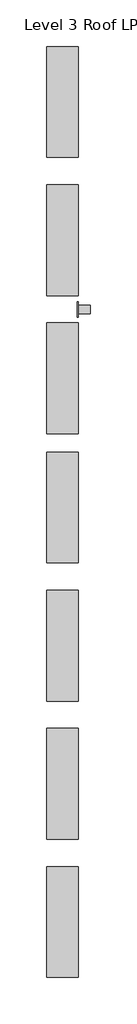
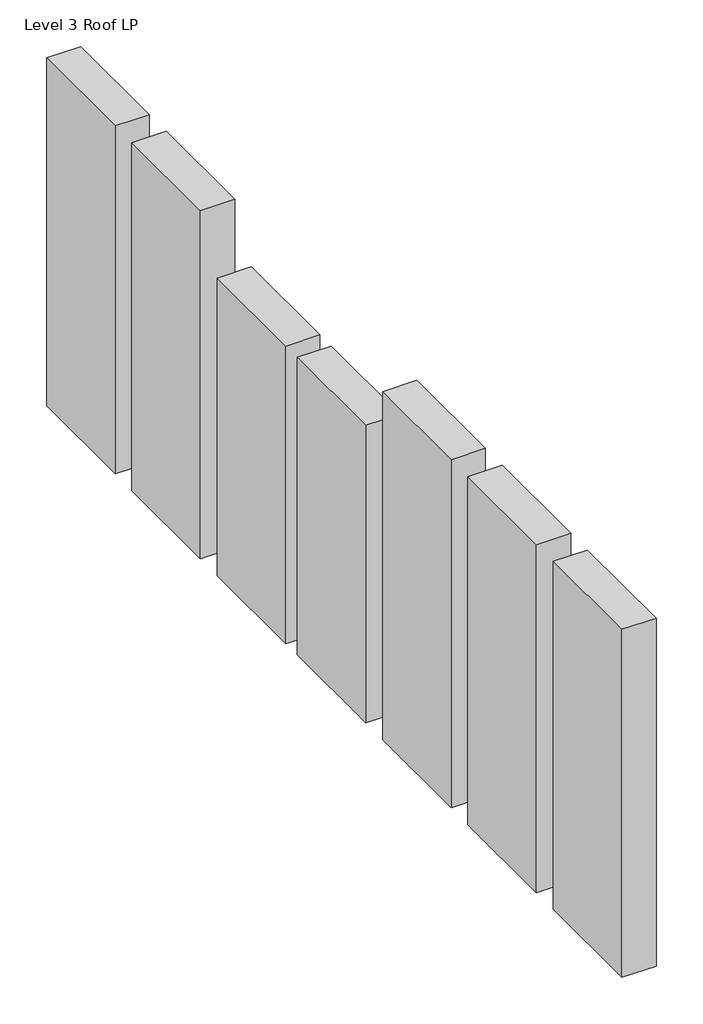
# One storey: 8 proxies.
"""IFC4 building model written with IfcOpenShell, lengths in millimetres."""

import ifcopenshell
import ifcopenshell.guid

model = None  # the IFC model being written
_history = None  # IfcOwnerHistory: only IFC2X3 demands one
_inside = {}  # id of a spatial element -> (the spatial element, [elements in it])
_under = {}  # id of a project, library or spatial element -> (it, [spatial elements below it])
_declared = {}  # id of a project -> (the project, [libraries it declares])
_typed = {}  # id of a type object -> (the type object, [elements of that type])
_made_of = {}  # id of a material, layer set ... -> (it, [elements and type objects made of it])


def new_model(schema):
    """Start an empty IFC model of exactly this schema.

    Asked for "IFC4X3", IfcOpenShell would pick the latest addendum, in which some entities
    have other attributes; the version numbers below select the first issue.
    IFC2X3 requires an IfcOwnerHistory on every rooted entity: one is made here for all.
    """
    global model, _history
    if schema == "IFC4X3":
        model = ifcopenshell.file(schema_version=(4, 3, 0, 0))
    else:
        model = ifcopenshell.file(schema=schema)
    _inside.clear()
    _under.clear()
    _declared.clear()
    _typed.clear()
    _made_of.clear()
    _history = None
    if model.schema == "IFC2X3":
        org = make("IfcOrganization", Name="unknown")
        user = make(
            "IfcPersonAndOrganization",
            ThePerson=make("IfcPerson", FamilyName="unknown"),
            TheOrganization=org,
        )
        app = make(
            "IfcApplication",
            ApplicationDeveloper=org,
            Version="unknown",
            ApplicationFullName="unknown",
            ApplicationIdentifier="unknown",
        )
        _history = make(
            "IfcOwnerHistory",
            OwningUser=user,
            OwningApplication=app,
            ChangeAction="ADDED",
            CreationDate=0,
        )
    return model


def make(cls, **values):
    """One entity of the class cls with the attributes given. An attribute that is None is left unset."""
    return model.create_entity(
        cls, **{name: value for name, value in values.items() if value is not None}
    )


def rooted(cls, **values):
    """An entity with a GlobalId (a new one), such as an element, a storey or a relation."""
    return make(cls, GlobalId=ifcopenshell.guid.new(), OwnerHistory=_history, **values)


def si_unit(unit_type, name, prefix=None):
    """IfcSIUnit, for example si_unit("LENGTHUNIT", "METRE", prefix="MILLI")."""
    return make("IfcSIUnit", UnitType=unit_type, Prefix=prefix, Name=name)


def assignment(units):
    """IfcUnitAssignment: the units of a project."""
    return None if units is None else make("IfcUnitAssignment", Units=units)


def point(xyz):
    """IfcCartesianPoint."""
    return None if xyz is None else make("IfcCartesianPoint", Coordinates=xyz)


def direction(xyz):
    """IfcDirection."""
    return None if xyz is None else make("IfcDirection", DirectionRatios=xyz)


def frame(location, z_axis=None, x_axis=None):
    """IfcAxis2Placement3D, a coordinate frame: its origin and axes. An axis left out is left unset."""
    return make(
        "IfcAxis2Placement3D",
        Location=point(location),
        Axis=direction(z_axis),
        RefDirection=direction(x_axis),
    )


def origin():
    """The frame at (0, 0, 0) with its axes left unset."""
    return frame((0.0, 0.0, 0.0))


def origin_with_axes():
    """The frame at (0, 0, 0) with the z axis (0, 0, 1) and the x axis (1, 0, 0) written out."""
    return frame((0.0, 0.0, 0.0), z_axis=(0.0, 0.0, 1.0), x_axis=(1.0, 0.0, 0.0))


def place(relative_to, where):
    """IfcLocalPlacement: puts the frame where relative to a parent placement (None: the world)."""
    return make(
        "IfcLocalPlacement", PlacementRelTo=relative_to, RelativePlacement=where
    )


def context(
    kind, dimensions, precision=None, world=None, true_north=None, identifier=None
):
    """IfcGeometricRepresentationContext, for example the 3D "Model" context."""
    return make(
        "IfcGeometricRepresentationContext",
        ContextIdentifier=identifier,
        ContextType=kind,
        CoordinateSpaceDimension=dimensions,
        Precision=precision,
        WorldCoordinateSystem=world,
        TrueNorth=true_north,
    )


def project(units=None, contexts=None):
    """IfcProject with its units and contexts."""
    return rooted(
        "IfcProject",
        Name="project",
        RepresentationContexts=contexts,
        UnitsInContext=assignment(units),
    )


def spatial(cls, under=None, at=None, **own):
    """A site, building, storey or space (cls), placed at a placement, below another one or the project."""
    s = rooted(cls, ObjectPlacement=at, **own)
    if under is not None:
        _under.setdefault(under.id(), (under, []))[1].append(s)
    return s


def polyline(points):
    """IfcPolyline through the points."""
    return make("IfcPolyline", Points=[point(p) for p in points])


def outline(outer, holes=None, kind="AREA"):
    """IfcArbitraryClosedProfileDef: a profile drawn as a closed curve; with holes, ...WithVoids."""
    if holes is None:
        return make("IfcArbitraryClosedProfileDef", ProfileType=kind, OuterCurve=outer)
    return make(
        "IfcArbitraryProfileDefWithVoids",
        ProfileType=kind,
        OuterCurve=outer,
        InnerCurves=holes,
    )


def extrude(swept, where, along, depth):
    """IfcExtrudedAreaSolid: the profile swept, set in the frame where, extruded along a direction by depth."""
    return make(
        "IfcExtrudedAreaSolid",
        SweptArea=swept,
        Position=where,
        ExtrudedDirection=direction(along),
        Depth=depth,
    )


def shape(context_of_items, identifier, shape_type, items):
    """IfcShapeRepresentation: the items that make up one representation, for example the "Body"."""
    return make(
        "IfcShapeRepresentation",
        ContextOfItems=context_of_items,
        RepresentationIdentifier=identifier,
        RepresentationType=shape_type,
        Items=items,
    )


def source(mapping_origin, context_of_items, identifier, shape_type, items):
    """IfcRepresentationMap: a shape defined once, which mapped items show again and again."""
    return make(
        "IfcRepresentationMap",
        MappingOrigin=mapping_origin,
        MappedRepresentation=shape(context_of_items, identifier, shape_type, items),
    )


def transform(
    local_origin,
    x_axis=None,
    y_axis=None,
    z_axis=None,
    scale=None,
    scale2=None,
    scale3=None,
    uniform=True,
):
    """IfcCartesianTransformationOperator3D, or its non-uniform kind. x_axis, y_axis, z_axis: its Axis1, 2, 3."""
    if uniform:
        return make(
            "IfcCartesianTransformationOperator3D",
            Axis1=direction(x_axis),
            Axis2=direction(y_axis),
            LocalOrigin=point(local_origin),
            Scale=scale,
            Axis3=direction(z_axis),
        )
    return make(
        "IfcCartesianTransformationOperator3DnonUniform",
        Axis1=direction(x_axis),
        Axis2=direction(y_axis),
        LocalOrigin=point(local_origin),
        Scale=scale,
        Axis3=direction(z_axis),
        Scale2=scale2,
        Scale3=scale3,
    )


def mapped(mapping_source, mapping_target):
    """IfcMappedItem: shows the shape of a source again, moved by a transform."""
    return make(
        "IfcMappedItem", MappingSource=mapping_source, MappingTarget=mapping_target
    )


def made_of(thing, what):
    """Note that an element or type object is made of a material, layer set ...; save() writes the relation."""
    if what is not None:
        _made_of.setdefault(what.id(), (what, []))[1].append(thing)
    return thing


def element(
    cls,
    number,
    at=None,
    inside=None,
    cuts=None,
    type_object=None,
    material=None,
    context=None,
    identifier="Body",
    shape_type=None,
    held_by="IfcProductDefinitionShape",
    body=None,
    shapes=None,
    **own,
):
    """One element of the class cls, such as IfcWall. Its Tag is "e" and its number.

    at: its placement. inside: the storey or other place that contains it. cuts: it is an
    opening in that element (IfcRelVoidsElement). A single representation is given by context,
    identifier, shape_type and body (its items); several are given by shapes. held_by: the class
    of the entity that holds the representations. save() writes the other relations.
    """
    e = rooted(cls, Tag="e%d" % number, ObjectPlacement=at, **own)
    if body is not None:
        shapes = [shape(context, identifier, shape_type, body)]
    if shapes is not None:
        e.Representation = make(held_by, Representations=shapes)
    if inside is not None:
        _inside.setdefault(inside.id(), (inside, []))[1].append(e)
    if cuts is not None:
        rooted(
            "IfcRelVoidsElement", RelatingBuildingElement=cuts, RelatedOpeningElement=e
        )
    if type_object is not None:
        _typed.setdefault(type_object.id(), (type_object, []))[1].append(e)
    return made_of(e, material)


def aggregate(whole, parts):
    """IfcRelAggregates: a whole, such as a stair, and the parts it consists of."""
    return rooted("IfcRelAggregates", RelatingObject=whole, RelatedObjects=parts)


def save(model, path):
    """Write the relations noted so far, then the file.

    IfcRelAggregates (storeys below a building ...), IfcRelContainedInSpatialStructure (elements
    in a storey), IfcRelDefinesByType, IfcRelAssociatesMaterial and IfcRelDeclares: one each for
    every whole, place, type object, material and project.
    """
    for whole, parts in _under.values():
        aggregate(whole, parts)
    for where, things in _inside.values():
        rooted(
            "IfcRelContainedInSpatialStructure",
            RelatedElements=things,
            RelatingStructure=where,
        )
    for kind, things in _typed.values():
        rooted("IfcRelDefinesByType", RelatedObjects=things, RelatingType=kind)
    for what, things in _made_of.values():
        rooted("IfcRelAssociatesMaterial", RelatedObjects=things, RelatingMaterial=what)
    for by, libraries in _declared.values():
        rooted("IfcRelDeclares", RelatingContext=by, RelatedDefinitions=libraries)
    model.write(path)


def emergency_lighting_distribution_board_600_a_cf68ca70(model_context):
    return source(origin(), model_context, "Body", "SweptSolid", [
        extrude(outline(polyline([(254.0, -1346.2), (-254.0, -1346.2), (-254.0, 0.0), (254.0, 0.0), (254.0, -1346.2)])), origin_with_axes(), (0.0, 0.0, 1.0), 146.1),
    ])


def lighting_and_appliance_panelboard_400v_mcb_surface_400_a_826206d9(model_context):
    return source(origin(), model_context, "Body", "SweptSolid", [
        extrude(outline(polyline([(254.0, -1574.8), (-254.0, -1574.8), (-254.0, 0.0), (254.0, 0.0), (254.0, -1574.8)])), origin_with_axes(), (0.0, 0.0, 1.0), 146.1),
    ])


def m_duplex_receptacle_top_switched_standard_10251bba(model_context):
    return source(origin(), model_context, "Body", "SweptSolid", [
        extrude(outline(polyline([(19.05, 38.1), (19.05, -38.1), (-19.05, -38.1), (-19.05, 38.1), (19.05, 38.1)])), frame((0.0, 0.0, -53.975), z_axis=(0.0, 0.0, 1.0), x_axis=(1.0, 0.0, 0.0)), (0.0, 0.0, 1.0), 53.975),
        extrude(outline(polyline([(34.925, 57.15), (34.925, -57.15), (-34.925, -57.15), (-34.925, 57.15), (34.925, 57.15)])), origin_with_axes(), (0.0, 0.0, 1.0), 4.7625),
    ])


model = new_model("IFC4")

# Units and contexts
model_context = context("Model", 3, world=origin())
ifc_project = project(units=[si_unit("LENGTHUNIT", "METRE", prefix="MILLI")], contexts=[model_context])

# Site, building, storey
site = spatial("IfcSite", under=ifc_project)
building = spatial("IfcBuilding", under=site)
storey = spatial("IfcBuildingStorey", under=building, Name="Level 3 Roof LP", Elevation=107300.0)

# Proxies
placement = place(None, origin())
emergency_lighting_distribution_board_600_a_shape = emergency_lighting_distribution_board_600_a_cf68ca70(model_context)
element("IfcBuildingElementProxy", 1, Name="Emergency Lighting Distribution Board : 600 A", ObjectType="Emergency Lighting Distribution Board : 600 A", at=placement, inside=storey, context=model_context, shape_type="MappedRepresentation", body=[
    mapped(emergency_lighting_distribution_board_600_a_shape, transform((15990.005, 12707.4241924, 101351.4), x_axis=(0.0, -1.0, 0.0), y_axis=(0.0, 0.0, 1.0), z_axis=(-1.0, 0.0, 0.0))),
])
element("IfcBuildingElementProxy", 2, Name="Emergency Lighting Distribution Board : 600 A", ObjectType="Emergency Lighting Distribution Board : 600 A", at=placement, inside=storey, context=model_context, shape_type="MappedRepresentation", body=[
    mapped(emergency_lighting_distribution_board_600_a_shape, transform((15990.005, 13299.4241924, 101351.4), x_axis=(0.0, -1.0, 0.0), y_axis=(0.0, 0.0, 1.0), z_axis=(-1.0, 0.0, 0.0))),
])
lighting_and_appliance_panelboard_400v_mcb_surface_400_a_shape = lighting_and_appliance_panelboard_400v_mcb_surface_400_a_826206d9(model_context)
element("IfcBuildingElementProxy", 3, Name="Lighting and Appliance Panelboard - 400V MCB - Surface : 400 A", ObjectType="Lighting and Appliance Panelboard - 400V MCB - Surface : 400 A", at=placement, inside=storey, context=model_context, shape_type="MappedRepresentation", body=[
    mapped(lighting_and_appliance_panelboard_400v_mcb_surface_400_a_shape, transform((15990.005, 10808.4241924, 101580.0), x_axis=(0.0, -1.0, 0.0), y_axis=(0.0, 0.0, 1.0), z_axis=(-1.0, 0.0, 0.0))),
])
element("IfcBuildingElementProxy", 4, Name="Lighting and Appliance Panelboard - 400V MCB - Surface : 400 A", ObjectType="Lighting and Appliance Panelboard - 400V MCB - Surface : 400 A", at=placement, inside=storey, context=model_context, shape_type="MappedRepresentation", body=[
    mapped(lighting_and_appliance_panelboard_400v_mcb_surface_400_a_shape, transform((15990.005, 11441.4241924, 101580.0), x_axis=(0.0, -1.0, 0.0), y_axis=(0.0, 0.0, 1.0), z_axis=(-1.0, 0.0, 0.0))),
])
element("IfcBuildingElementProxy", 5, Name="Lighting and Appliance Panelboard - 400V MCB - Surface : 400 A", ObjectType="Lighting and Appliance Panelboard - 400V MCB - Surface : 400 A", at=placement, inside=storey, context=model_context, shape_type="MappedRepresentation", body=[
    mapped(lighting_and_appliance_panelboard_400v_mcb_surface_400_a_shape, transform((15990.005, 12074.4241924, 101580.0), x_axis=(0.0, -1.0, 0.0), y_axis=(0.0, 0.0, 1.0), z_axis=(-1.0, 0.0, 0.0))),
])
element("IfcBuildingElementProxy", 6, Name="Lighting and Appliance Panelboard - 400V MCB - Surface : 400 A", ObjectType="Lighting and Appliance Panelboard - 400V MCB - Surface : 400 A", at=placement, inside=storey, context=model_context, shape_type="MappedRepresentation", body=[
    mapped(lighting_and_appliance_panelboard_400v_mcb_surface_400_a_shape, transform((15990.005, 13932.4241924, 101580.0), x_axis=(0.0, -1.0, 0.0), y_axis=(0.0, 0.0, 1.0), z_axis=(-1.0, 0.0, 0.0))),
])
element("IfcBuildingElementProxy", 7, Name="Lighting and Appliance Panelboard - 400V MCB - Surface : 400 A", ObjectType="Lighting and Appliance Panelboard - 400V MCB - Surface : 400 A", at=placement, inside=storey, context=model_context, shape_type="MappedRepresentation", body=[
    mapped(lighting_and_appliance_panelboard_400v_mcb_surface_400_a_shape, transform((15990.005, 14565.4241924, 101580.0), x_axis=(0.0, -1.0, 0.0), y_axis=(0.0, 0.0, 1.0), z_axis=(-1.0, 0.0, 0.0))),
])
m_duplex_receptacle_top_switched_standard_shape = m_duplex_receptacle_top_switched_standard_10251bba(model_context)
element("IfcBuildingElementProxy", 8, Name="M_Receptacle - 220V : Standard", ObjectType="M_Receptacle - 220V : Standard", at=placement, inside=storey, context=model_context, shape_type="MappedRepresentation", body=[
    mapped(m_duplex_receptacle_top_switched_standard_shape, transform((15990.005, 13614.2932067, 100325.120044), x_axis=(0.0, -1.0, 0.0), y_axis=(0.0, 0.0, 1.0), z_axis=(-1.0, 0.0, 0.0))),
])

save(model, "model.ifc")

# Revit data of these elements
# Type "Emergency Lighting Distribution Board : 600 A"
#   Type Mark = "Emergency Lighting Distribution Board"
#   Classification.OmniClass.21.Number = "21-04 50 40 50"
#   Classification.OmniClass.21.Description = "Lighting Fixtures"
#   Classification.UniFormat.II.Description = "Lighting Fixtures"
#   Classification.OmniClass.23.Number = "23-35 31 13"
#   Classification.OmniClass.23.Description = "Distribution Panel Boards"
#   Classification.UniFormat.II.Number = "D5040.50"
#   COBie.Type.CreatedBy = "info@mma.ie"
#   COBie.Type.CreatedOn = "2017-07-25T10:15:16"
#   COBie.Type.Name = "Emergency Lighting Distribution Board"
#   COBie.Type.Category = "23-35 31 13 : Distribution Panel Boards"
#   COBie.Type.Description = "Emergency Lighting Distribution Board_600 A"
#   COBie.Type.AssetType = "Fixed"
#   COBie.Type.Manufacturer = ""
#   COBie.Type.ModelNumber = ""
#   Wattage = "400"
#   Voltage = "600"
#   built-in parameter 1140081 [instance default] = "Recessed"
#   Keynote = "26 26 00.A"
#   built-in parameter 1140083 [instance default] = "Type 1"
#   COBie.Type.ReplacementCost = 0
#   Width = 508 mm
#   built-in parameter 1140082 [instance default] = 100 (stored number, unit not read)
#   built-in parameter 1140140 [instance default] = 600 (stored number, unit not read)
#   Height [instance default] = 1346.2 mm
#   ELDB Width = 508 mm
#   ELDB Height = 1346.2 mm
#   ELDB Depth = 146.1 mm
#   Depth = 146.1 mm
#   Default Elevation = 1200 mm
#   Ballast Wattage = 400 W
#   Ballast Voltage = 600 V
#   42 Circuit Height = 1879.6 mm
#   30 Circuit Height = 1651 mm
#   24 Circuit Height = 1346.2 mm
#   12 Circuit Height = 1346.2 mm
#   COBie.Type = yes
#   built-in parameter 1140142 [instance default] = -1
#   built-in parameter 1140079 [instance default] = 12
#   built-in parameter 1155100 [instance default] = -1
#   Load Classification = Other
# Type "Lighting and Appliance Panelboard - 400V MCB - Surface : 400 A"
#   Type Mark = "Lighting and Appliance Panelboard - 400V MCB - Surface"
#   Classification.OmniClass.21.Number = "21-04 50 30 50"
#   Classification.MasterFormat.Description = "Wiring Devices"
#   Classification.OmniClass.22.Number = "22-26 27 26"
#   Classification.OmniClass.21.Description = "Wiring Devices"
#   Classification.UniFormat.II.Description = "Wiring Devices"
#   Classification.MasterFormat.Number = "26 27 26"
#   Classification.OmniClass.23.Number = "23-35 31 29"
#   Classification.OmniClass.22.Description = "Wiring Devices"
#   Classification.OmniClass.23.Description = "Switchboards"
#   Classification.UniFormat.II.Number = "D5030.50"
#   COBie.Type.CreatedBy = "info@mma.ie"
#   COBie.Type.CreatedOn = "2017-07-25T10:15:16"
#   COBie.Type.Name = "Lighting and Appliance Panelboard - 400V MCB - Surface"
#   COBie.Type.Category = "23-35 31 29 : Switchboards"
#   COBie.Type.Description = "Lighting and Appliance Panelboard - 400V MCB - Surface_400 A"
#   COBie.Type.AssetType = "Fixed"
#   COBie.Type.Manufacturer = ""
#   COBie.Type.ModelNumber = ""
#   Wattage = "400"
#   Voltage = "600"
#   built-in parameter 1140081 [instance default] = "Surface"
#   Keynote = "26 24 16.A"
#   built-in parameter 1140083 [instance default] = "Type 1"
#   COBie.Type.ReplacementCost = 0
#   Width = 508 mm
#   built-in parameter 1140082 [instance default] = 100 (stored number, unit not read)
#   built-in parameter 1140140 [instance default] = 400 (stored number, unit not read)
#   L.A.P. Width = 508 mm
#   L.A.P. Height = 1574.8 mm
#   L.A.P. Depth = 146.1 mm
#   Height [instance default] = 1574.8 mm
#   Depth = 146.1 mm
#   Default Elevation = 1200 mm
#   Ballast Wattage = 400 W
#   Ballast Voltage = 600 V
#   42 Circuit Height = 1727.2 mm
#   30 Circuit Height = 1574.8 mm
#   18 Circuit Height = 1574.8 mm
#   12 Circuit Height = 1574.8 mm
#   COBie.Type = yes
#   built-in parameter 1140142 [instance default] = -1
#   built-in parameter 1140079 [instance default] = 12
#   built-in parameter 1155100 [instance default] = -1
#   Load Classification = Other
# Type "M_Receptacle - 220V : Standard"
#   Type Mark = "M_Receptacle - 220V"
#   Classification.OmniClass.21.Number = "21-04 50 30 50"
#   Classification.MasterFormat.Description = "Wiring Devices"
#   Classification.OmniClass.22.Number = "22-26 27 26"
#   Classification.OmniClass.21.Description = "Wiring Devices"
#   Classification.UniFormat.II.Description = "Wiring Devices"
#   Classification.MasterFormat.Number = "26 27 26"
#   Classification.OmniClass.23.Number = "23-35 27 11"
#   Classification.OmniClass.22.Description = "Wiring Devices"
#   Classification.OmniClass.23.Description = "Electrical Receptacles"
#   Classification.UniFormat.II.Number = "D5030.50"
#   COBie.Type.CreatedBy = "info@mma.ie"
#   COBie.Type.CreatedOn = "2017-07-25T10:15:16"
#   COBie.Type.Name = "M_Receptacle - 220V"
#   COBie.Type.Category = "23-35 27 11 : Electrical Receptacles"
#   COBie.Type.Description = "M_Receptacle - 220V_Standard"
#   COBie.Type.AssetType = "Fixed"
#   COBie.Type.Manufacturer = ""
#   COBie.Type.ModelNumber = ""
#   Keynote = "26 27 26.D"
#   COBie.Type.ReplacementCost = 0
#   Switch Voltage = 220 V
#   Recep.Width [instance default] = 69.85 mm
#   Recep.Load = 180 VA
#   Recep.Height [instance default] = 114.3 mm
#   Load = 180 VA
#   Default Elevation = 460 mm
#   COBie.Type = yes
#   Recep.Material = Stainless Steel
#   Load Classification = Receptacle
#   Assembly Code = ""
# Element 1 (IfcBuildingElementProxy, "Emergency Lighting Distribution Board : 600 A")
#   Panel Name = "EM.P2"
#   Comments = "EM.P2"
#   Mark = "1"
#   COBie.CreatedBy = "info@mma.ie"
#   COBie.CreatedOn = "2017-07-25T10:15:16"
#   COBie.Component.Name = "Emergency Lighting Distribution Board_1"
#   COBie.Component.Space = "105"
#   COBie.Component.Description = "Emergency Lighting Distribution Board: 600 A"
#   Notes = "n/a"
#   Floor Level = "Level 1"
#   built-in parameter 1140081 = "Recessed"
#   built-in parameter 1140083 = "Type 1"
#   built-in parameter 1140082 = 100 (stored number, unit not read)
#   built-in parameter 1140140 = 600 (stored number, unit not read)
#   Height = 1346.2 mm
#   COBie = yes
#   built-in parameter 1140079 = 12
#   built-in parameter 1140064 = 230/400 Wye
#   Phase Created = New Construction
# Element 2 (IfcBuildingElementProxy, "Emergency Lighting Distribution Board : 600 A")
#   Panel Name = "EM.P1"
#   Comments = ""
#   Mark = "2"
#   COBie.CreatedBy = "info@mma.ie"
#   COBie.CreatedOn = "2017-07-25T10:15:16"
#   COBie.Component.Name = "Emergency Lighting Distribution Board_2"
#   COBie.Component.Space = "105"
#   COBie.Component.Description = "Emergency Lighting Distribution Board: 600 A"
#   Notes = "n/a"
#   Floor Level = "Level 1"
#   built-in parameter 1140081 = "Recessed"
#   built-in parameter 1140083 = "Type 1"
#   built-in parameter 1140082 = 100 (stored number, unit not read)
#   built-in parameter 1140140 = 600 (stored number, unit not read)
#   Height = 1346.2 mm
#   COBie = yes
#   built-in parameter 1140079 = 12
#   built-in parameter 1140064 = 230/400 Wye
#   Phase Created = New Construction
# Element 3 (IfcBuildingElementProxy, "Lighting and Appliance Panelboard - 400V MCB - Surface : 400 A")
#   Panel Name = "EP3"
#   Comments = "EP3"
#   Mark = "1"
#   COBie.CreatedBy = "info@mma.ie"
#   COBie.CreatedOn = "2017-07-25T10:15:16"
#   COBie.Component.Name = "Lighting and Appliance Panelboard - 400V MCB - Surface_1"
#   COBie.Component.Space = "105"
#   COBie.Component.Description = "Lighting and Appliance Panelboard - 400V MCB - Surface: 400 A"
#   Notes = "n/a"
#   Floor Level = "Level 1"
#   built-in parameter 1140081 = "Surface"
#   built-in parameter 1140083 = "Type 1"
#   built-in parameter 1140082 = 100 (stored number, unit not read)
#   built-in parameter 1140140 = 400 (stored number, unit not read)
#   Height = 1574.8 mm
#   COBie = yes
#   built-in parameter 1140079 = 12
#   built-in parameter 1140064 = 230/400 Wye
#   Phase Created = New Construction
# Element 4 (IfcBuildingElementProxy, "Lighting and Appliance Panelboard - 400V MCB - Surface : 400 A")
#   Panel Name = "EP2"
#   Comments = "EP2"
#   Mark = "2"
#   COBie.CreatedBy = "info@mma.ie"
#   COBie.CreatedOn = "2017-07-25T10:15:16"
#   COBie.Component.Name = "Lighting and Appliance Panelboard - 400V MCB - Surface_2"
#   COBie.Component.Space = "105"
#   COBie.Component.Description = "Lighting and Appliance Panelboard - 400V MCB - Surface: 400 A"
#   Notes = "n/a"
#   Floor Level = "Level 1"
#   built-in parameter 1140081 = "Surface"
#   built-in parameter 1140083 = "Type 1"
#   built-in parameter 1140082 = 100 (stored number, unit not read)
#   built-in parameter 1140140 = 400 (stored number, unit not read)
#   Height = 1574.8 mm
#   COBie = yes
#   built-in parameter 1140079 = 12
#   built-in parameter 1140064 = 230/400 Wye
#   Phase Created = New Construction
# Element 5 (IfcBuildingElementProxy, "Lighting and Appliance Panelboard - 400V MCB - Surface : 400 A")
#   Panel Name = "EP1"
#   Comments = "EP1"
#   Mark = "3"
#   COBie.CreatedBy = "info@mma.ie"
#   COBie.CreatedOn = "2017-07-25T10:15:16"
#   COBie.Component.Name = "Lighting and Appliance Panelboard - 400V MCB - Surface_3"
#   COBie.Component.Space = "105"
#   COBie.Component.Description = "Lighting and Appliance Panelboard - 400V MCB - Surface: 400 A"
#   Notes = "n/a"
#   Floor Level = "Level 1"
#   built-in parameter 1140081 = "Surface"
#   built-in parameter 1140083 = "Type 1"
#   built-in parameter 1140082 = 100 (stored number, unit not read)
#   built-in parameter 1140140 = 400 (stored number, unit not read)
#   Height = 1574.8 mm
#   COBie = yes
#   built-in parameter 1140079 = 12
#   built-in parameter 1140064 = 230/400 Wye
#   Phase Created = New Construction
# Element 6 (IfcBuildingElementProxy, "Lighting and Appliance Panelboard - 400V MCB - Surface : 400 A")
#   Panel Name = "EP4"
#   Comments = "EP4"
#   Mark = "4"
#   COBie.CreatedBy = "info@mma.ie"
#   COBie.CreatedOn = "2017-07-25T10:15:16"
#   COBie.Component.Name = "Lighting and Appliance Panelboard - 400V MCB - Surface_4"
#   COBie.Component.Space = "105"
#   COBie.Component.Description = "Lighting and Appliance Panelboard - 400V MCB - Surface: 400 A"
#   Notes = "n/a"
#   built-in parameter 1140081 = "Surface"
#   built-in parameter 1140083 = "Type 1"
#   built-in parameter 1140082 = 100 (stored number, unit not read)
#   built-in parameter 1140140 = 400 (stored number, unit not read)
#   Height = 1574.8 mm
#   COBie = yes
#   built-in parameter 1140079 = 12
#   built-in parameter 1140064 = 230/400 Wye
#   Phase Created = New Construction
# Element 7 (IfcBuildingElementProxy, "Lighting and Appliance Panelboard - 400V MCB - Surface : 400 A")
#   Panel Name = "EP5"
#   Comments = "EP5"
#   Mark = "5"
#   COBie.CreatedBy = "info@mma.ie"
#   COBie.CreatedOn = "2017-07-25T10:15:16"
#   COBie.Component.Name = "Lighting and Appliance Panelboard - 400V MCB - Surface_5"
#   COBie.Component.Space = "105"
#   COBie.Component.Description = "Lighting and Appliance Panelboard - 400V MCB - Surface: 400 A"
#   Notes = "n/a"
#   built-in parameter 1140081 = "Surface"
#   built-in parameter 1140083 = "Type 1"
#   built-in parameter 1140082 = 100 (stored number, unit not read)
#   built-in parameter 1140140 = 400 (stored number, unit not read)
#   Height = 1574.8 mm
#   COBie = yes
#   built-in parameter 1140079 = 12
#   built-in parameter 1140064 = 230/400 Wye
#   Phase Created = New Construction
# Element 8 (IfcBuildingElementProxy, "M_Receptacle - 220V : Standard")
#   Mark = "59"
#   COBie.CreatedBy = "info@mma.ie"
#   COBie.CreatedOn = "2017-07-25T10:15:16"
#   COBie.Component.Name = "M_Receptacle - 220V_59"
#   COBie.Component.Space = "105"
#   COBie.Component.Description = "M_Receptacle - 220V: Standard"
#   Notes = "n/a"
#   COBie = yes
#   Phase Created = New Construction
# Materials
#   "Stainless Steel": class "Metal", colour RGB 120 120 120, transparency 0, Description = "Stainless Steel 18/8", Cost = 0
# Space at (17805.746, 10558.313) mm, phase "New Construction", upper level "Level 3 Roof LP", upper offset 2000 mm, lower offset 0 mm
#   Number = "301"
#   Name = "Roof Space Level 3"
#   Classification.Space.Number = "13-69 13"
#   Classification.Space.Description = "Roof Terrace"
#   COBie.CreatedBy = "info@mma.ie"
#   COBie.CreatedOn = "2017-07-25T10:15:16"
#   COBie.Space.Name = "301"
#   COBie.Space.Category = "13-69 13 : Roof Terraces"
#   COBie.Space.Description = "Roof Terrace"
#   Actual Lighting Load per area = 0
#   Actual Power Load per area = 0
#   Sensible Heat Gain per person = 0
#   Specified Lighting Load = 0
#   Specified Power Load = 0
#   Latent Heat Gain per person = 0
#   Total Heat Gain per person = 0
#   Area per Person = 0
#   Number of People = 11.1605 (stored number, unit not read)
#   COBie.Space.UsableHeight = 2000 mm
#   COBie.Space.GrossArea = 315.053 m²
#   COBie.Space.NetArea = 0 m²
#   Lighting Load Units = 0
#   Power Load Units = 0
#   Return Airflow = 0
#   Occupancy Unit = -1
#   Condition Type = 2
#   COBie = yes
#   Construction Type = none
